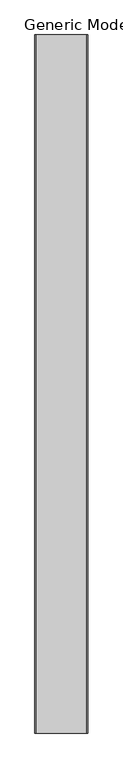
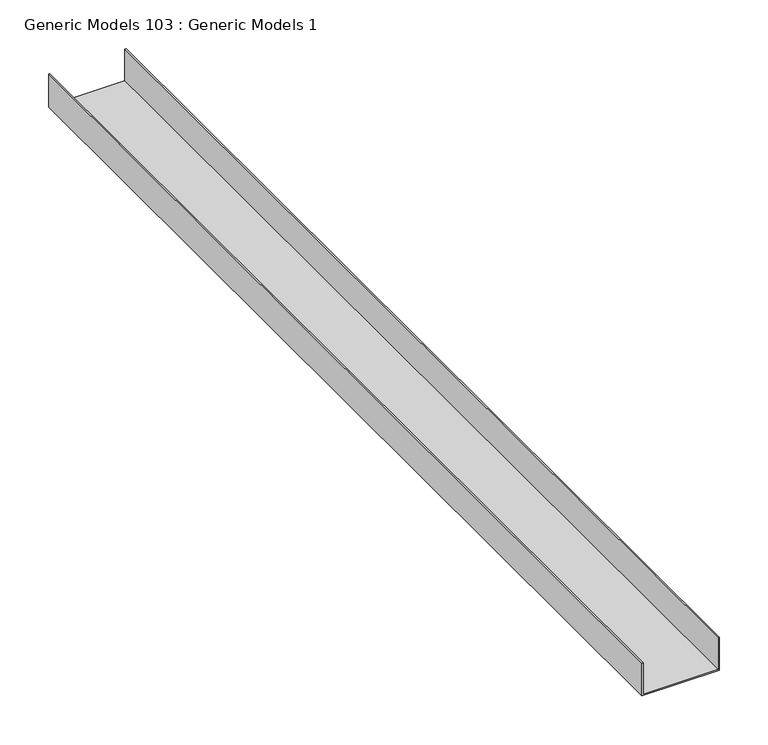
"""IFC4 building model written with IfcOpenShell, lengths in millimetres: proxy geometry, Generic Models 103 : Generic Models 1."""

from ifc_helpers import new_model, si_unit, frame, origin, place, context, project, spatial, polyline, outline, extrude, source, transform, mapped, element, save


def generic_models_103_generic_models_1_38d4618c(model_context):
    return source(origin(), model_context, "Body", "SweptSolid", [
        extrude(outline(polyline([(0.0, 49784.0), (41.275, 49784.0), (41.275, 49782.4125), (1.5875, 49782.4125), (1.5875, 49693.5125), (41.275, 49693.5125), (41.275, 49691.925), (0.0, 49691.925), (0.0, 49784.0)])), frame((0.0, 0.0, 0.0), z_axis=(0.0, 1.0, 0.0), x_axis=(0.0, 0.0, 1.0)), (0.0, 0.0, 1.0), 1219.2),
    ])


if __name__ == "__main__":
    model = new_model("IFC4")
    model_context = context("Model", 3, world=origin())
    ifc_project = project(units=[si_unit("LENGTHUNIT", "METRE", prefix="MILLI")], contexts=[model_context])
    site = spatial("IfcSite", under=ifc_project)
    building = spatial("IfcBuilding", under=site)
    placement = place(None, origin())
    generic_models_103_generic_models_1_shape = generic_models_103_generic_models_1_38d4618c(model_context)
    element("IfcBuildingElementProxy", 1, Name="Generic Models 103 : Generic Models 1", ObjectType="Generic Models 103 : Generic Models 1", at=placement, inside=building, context=model_context, shape_type="MappedRepresentation", body=[
        mapped(generic_models_103_generic_models_1_shape, transform((0.0, 0.0, 0.0), x_axis=(1.0, 0.0, 0.0), y_axis=(0.0, 1.0, 0.0), z_axis=(0.0, 0.0, 1.0))),
    ])
    save(model, "model.ifc")

# Revit data of these elements
# Element 1 (IfcBuildingElementProxy, "Generic Models 103 : Generic Models 1")
#   Materials on its faces: "METAL RUNNER ANCHORED TO STRUCTURE"
# Materials
#   "METAL RUNNER ANCHORED TO STRUCTURE": class "Unassigned", colour RGB 210 209 208, transparency 0, Keynote = "M05121300.02", Cost = 0
